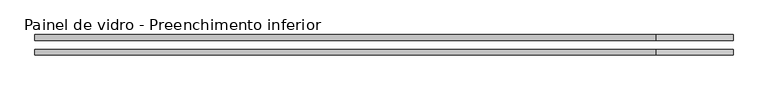
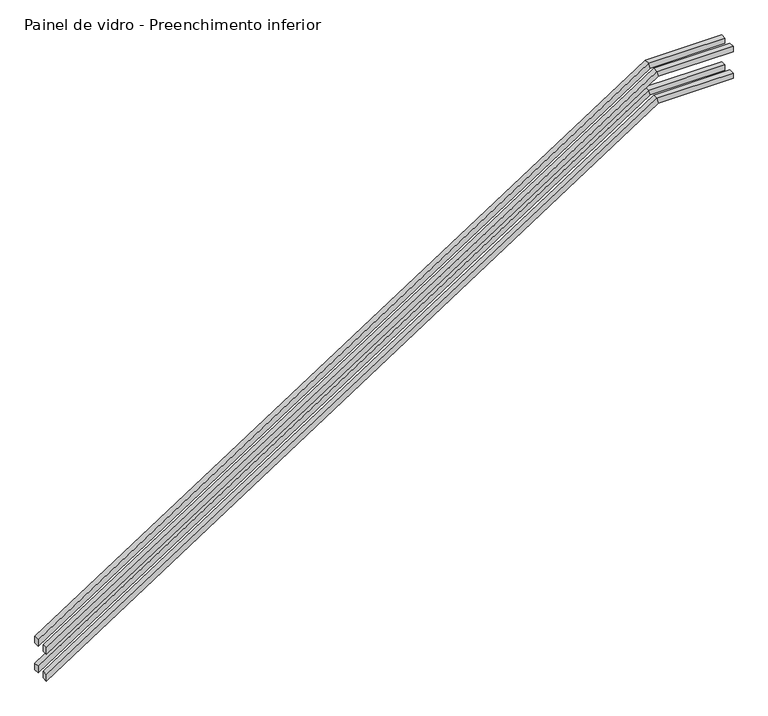
"""IFC4 building model written with IfcOpenShell, lengths in millimetres: railing geometry, Painel de vidro - Preenchimento inferior."""

from ifc_helpers import new_model, si_unit, origin, place, context, project, spatial, faceted_brep, source, transform, mapped, element, save


def painel_de_vidro_preenchimento_inferior_9d6dc48f(model_context):
    return source(origin(), model_context, "Body", "Brep", [
        faceted_brep([(8329.9999996, 4463.4, 2675.0), (8329.9999996, 4463.4, 2655.0), (8329.9999996, 4483.4, 2655.0), (8329.9999996, 4483.4, 2675.0), (8059.9999996, 4463.4, 2675.0), (8065.9146294, 4463.4, 2655.0), (8065.9146294, 4483.4, 2655.0), (8059.9999996, 4483.4, 2675.0), (5899.9999996, 4463.4, 1275.0), (5899.9999996, 4483.4, 1275.0), (5899.9999996, 4483.4, 1251.1664436), (5899.9999996, 4463.4, 1251.1664436)], [[[0, 1, 2, 3]], [[1, 0, 4, 5]], [[2, 1, 5, 6]], [[3, 2, 6, 7]], [[0, 3, 7, 4]], [[8, 9, 10, 11]], [[5, 4, 8, 11]], [[6, 5, 11, 10]], [[7, 6, 10, 9]], [[4, 7, 9, 8]]]),
        faceted_brep([(5899.9999996, 4432.6, 1275.0), (5899.9999996, 4432.6, 1251.1664436), (5899.9999996, 4412.6, 1251.1664436), (5899.9999996, 4412.6, 1275.0), (8059.9999996, 4432.6, 2675.0), (8065.9146294, 4432.6, 2655.0), (8065.9146294, 4412.6, 2655.0), (8059.9999996, 4412.6, 2675.0), (8329.9999996, 4432.6, 2675.0), (8329.9999996, 4412.6, 2675.0), (8329.9999996, 4412.6, 2655.0), (8329.9999996, 4432.6, 2655.0)], [[[0, 1, 2, 3]], [[1, 0, 4, 5]], [[2, 1, 5, 6]], [[3, 2, 6, 7]], [[0, 3, 7, 4]], [[8, 9, 10, 11]], [[5, 4, 8, 11]], [[6, 5, 11, 10]], [[7, 6, 10, 9]], [[4, 7, 9, 8]]]),
        faceted_brep([(8329.9999996, 4463.4, 2575.0), (8329.9999996, 4463.4, 2555.0), (8329.9999996, 4483.4, 2555.0), (8329.9999996, 4483.4, 2575.0), (8059.9999996, 4463.4, 2575.0), (8065.9146294, 4463.4, 2555.0), (8065.9146294, 4483.4, 2555.0), (8059.9999996, 4483.4, 2575.0), (5899.9999996, 4463.4, 1175.0), (5899.9999996, 4483.4, 1175.0), (5899.9999996, 4483.4, 1151.1664436), (5899.9999996, 4463.4, 1151.1664436)], [[[0, 1, 2, 3]], [[1, 0, 4, 5]], [[2, 1, 5, 6]], [[3, 2, 6, 7]], [[0, 3, 7, 4]], [[8, 9, 10, 11]], [[5, 4, 8, 11]], [[6, 5, 11, 10]], [[7, 6, 10, 9]], [[4, 7, 9, 8]]]),
        faceted_brep([(5899.9999996, 4432.6, 1175.0), (5899.9999996, 4432.6, 1151.1664436), (5899.9999996, 4412.6, 1151.1664436), (5899.9999996, 4412.6, 1175.0), (8059.9999996, 4432.6, 2575.0), (8065.9146294, 4432.6, 2555.0), (8065.9146294, 4412.6, 2555.0), (8059.9999996, 4412.6, 2575.0), (8329.9999996, 4432.6, 2575.0), (8329.9999996, 4412.6, 2575.0), (8329.9999996, 4412.6, 2555.0), (8329.9999996, 4432.6, 2555.0)], [[[0, 1, 2, 3]], [[1, 0, 4, 5]], [[2, 1, 5, 6]], [[3, 2, 6, 7]], [[0, 3, 7, 4]], [[8, 9, 10, 11]], [[5, 4, 8, 11]], [[6, 5, 11, 10]], [[7, 6, 10, 9]], [[4, 7, 9, 8]]]),
    ])


if __name__ == "__main__":
    model = new_model("IFC4")
    model_context = context("Model", 3, world=origin())
    ifc_project = project(units=[si_unit("LENGTHUNIT", "METRE", prefix="MILLI")], contexts=[model_context])
    site = spatial("IfcSite", under=ifc_project)
    building = spatial("IfcBuilding", under=site)
    placement = place(None, origin())
    painel_de_vidro_preenchimento_inferior_shape = painel_de_vidro_preenchimento_inferior_9d6dc48f(model_context)
    element("IfcRailing", 1, ObjectType="Painel de vidro - Preenchimento inferior", at=placement, inside=building, context=model_context, shape_type="MappedRepresentation", body=[
        mapped(painel_de_vidro_preenchimento_inferior_shape, transform((0.0, 0.0, 0.0), x_axis=(1.0, 0.0, 0.0), y_axis=(0.0, 1.0, 0.0), z_axis=(0.0, 0.0, 1.0))),
    ])
    save(model, "model.ifc")
